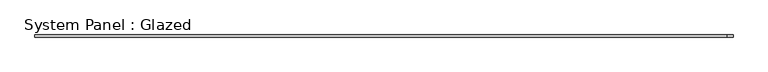
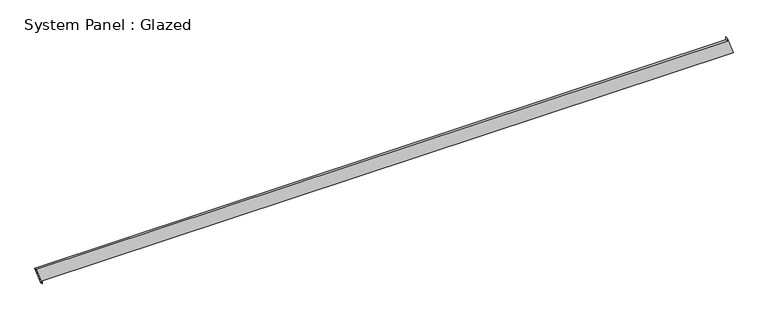
"""IFC4 building model written with IfcOpenShell, lengths in millimetres: plate geometry, System Panel : Glazed."""

from ifc_helpers import new_model, si_unit, frame, origin, place, context, project, spatial, polyline, outline, extrude, source, transform, mapped, element, save


def system_panel_glazed_d1cd71b4(model_context):
    return source(origin(), model_context, "Body", "SweptSolid", [
        extrude(outline(polyline([(0.0, -3958.4083386), (35.3553391, -3958.4083386), (35.3553391, 4027.6365543), (235.670353, 3958.7537794), (200.315014, 3958.7544121), (200.1720966, -4027.6365543), (0.0, -3958.4083386)])), frame((0.0, -49.5, 0.0), z_axis=(0.0, 1.0, 0.0), x_axis=(0.0, 0.0, 1.0)), (0.0, 0.0, 1.0), 25.0),
    ])


if __name__ == "__main__":
    model = new_model("IFC4")
    model_context = context("Model", 3, world=origin())
    ifc_project = project(units=[si_unit("LENGTHUNIT", "METRE", prefix="MILLI")], contexts=[model_context])
    site = spatial("IfcSite", under=ifc_project)
    building = spatial("IfcBuilding", under=site)
    placement = place(None, origin())
    system_panel_glazed_shape = system_panel_glazed_d1cd71b4(model_context)
    element("IfcPlate", 1, ObjectType="System Panel : Glazed", at=placement, inside=building, context=model_context, shape_type="MappedRepresentation", body=[
        mapped(system_panel_glazed_shape, transform((0.0, 0.0, 0.0), x_axis=(1.0, 0.0, 0.0), y_axis=(0.0, 1.0, 0.0), z_axis=(0.0, 0.0, 1.0))),
    ])
    save(model, "model.ifc")

# Revit data of these elements
# Element 1 (IfcPlate, "System Panel : Glazed")
#   Materials on its faces: "Glass"
# Materials
#   "Glass": class "Glass", colour RGB 218 227 224, transparency 0.85, Description = "Soda Lime Glass", Cost = 0
